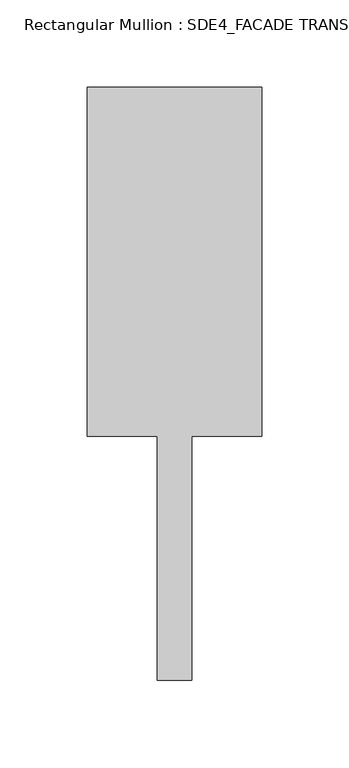
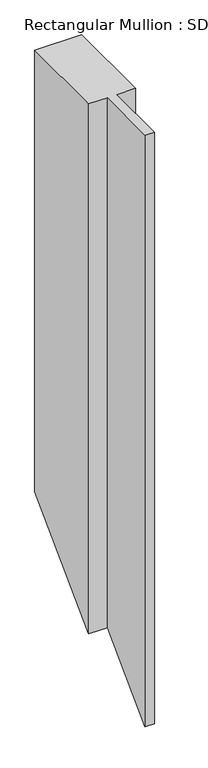
"""IFC4 building model written with IfcOpenShell, lengths in millimetres: member geometry, Rectangular Mullion : SDE4_FACADE TRANSOM TYPE 1."""

from ifc_helpers import new_model, si_unit, origin, place, context, project, spatial, faceted_brep, source, transform, mapped, element, save


def rectangular_mullion_sde4_facade_transom_type_1_b3cdbbc7(model_context):
    return source(origin(), model_context, "Body", "Brep", [
        faceted_brep([(50.0, 132.5, 0.0), (-50.0, 132.5, 0.0), (-50.0, -67.5, 0.0), (-10.0, -67.5, 0.0), (-10.0, -207.5, 0.0), (10.0, -207.5, 0.0), (10.0, -67.5, 0.0), (50.0, -67.5, 0.0), (50.0, 132.5, -999.0000001), (-50.0, 132.5, -999.0000001), (-50.0, -67.5, -1199.0000001), (-10.0, -67.5, -1199.0000001), (-10.0, -207.5, -1339.0000001), (10.0, -207.5, -1339.0000001), (10.0, -67.5, -1199.0000001), (50.0, -67.5, -1199.0000001)], [[[0, 1, 2, 3, 4, 5, 6, 7]], [[1, 0, 8, 9]], [[2, 1, 9, 10]], [[3, 2, 10, 11]], [[4, 3, 11, 12]], [[5, 4, 12, 13]], [[6, 5, 13, 14]], [[7, 6, 14, 15]], [[0, 7, 15, 8]], [[8, 15, 14, 13, 12, 11, 10, 9]]]),
    ])


if __name__ == "__main__":
    model = new_model("IFC4")
    model_context = context("Model", 3, world=origin())
    ifc_project = project(units=[si_unit("LENGTHUNIT", "METRE", prefix="MILLI")], contexts=[model_context])
    site = spatial("IfcSite", under=ifc_project)
    building = spatial("IfcBuilding", under=site)
    placement = place(None, origin())
    rectangular_mullion_sde4_facade_transom_type_1_shape = rectangular_mullion_sde4_facade_transom_type_1_b3cdbbc7(model_context)
    element("IfcMember", 1, ObjectType="Rectangular Mullion : SDE4_FACADE TRANSOM TYPE 1", at=placement, inside=building, context=model_context, shape_type="MappedRepresentation", body=[
        mapped(rectangular_mullion_sde4_facade_transom_type_1_shape, transform((0.0, 0.0, 0.0), x_axis=(1.0, 0.0, 0.0), y_axis=(0.0, 1.0, 0.0), z_axis=(0.0, 0.0, 1.0))),
    ])
    save(model, "model.ifc")

# Revit data of these elements
# Type "Rectangular Mullion : SDE4_FACADE TRANSOM TYPE 1"
#   built-in parameter 1007322 = 1.11549 (stored number, unit not read)
#   built-in parameter 1007321 = 0.164042 (stored number, unit not read)
#   built-in parameter 1007320 = 0.164042 (stored number, unit not read)
